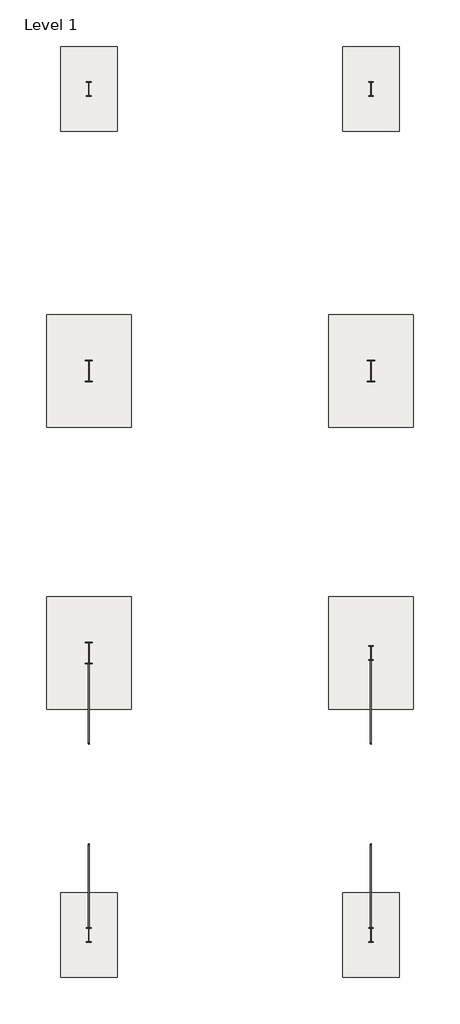
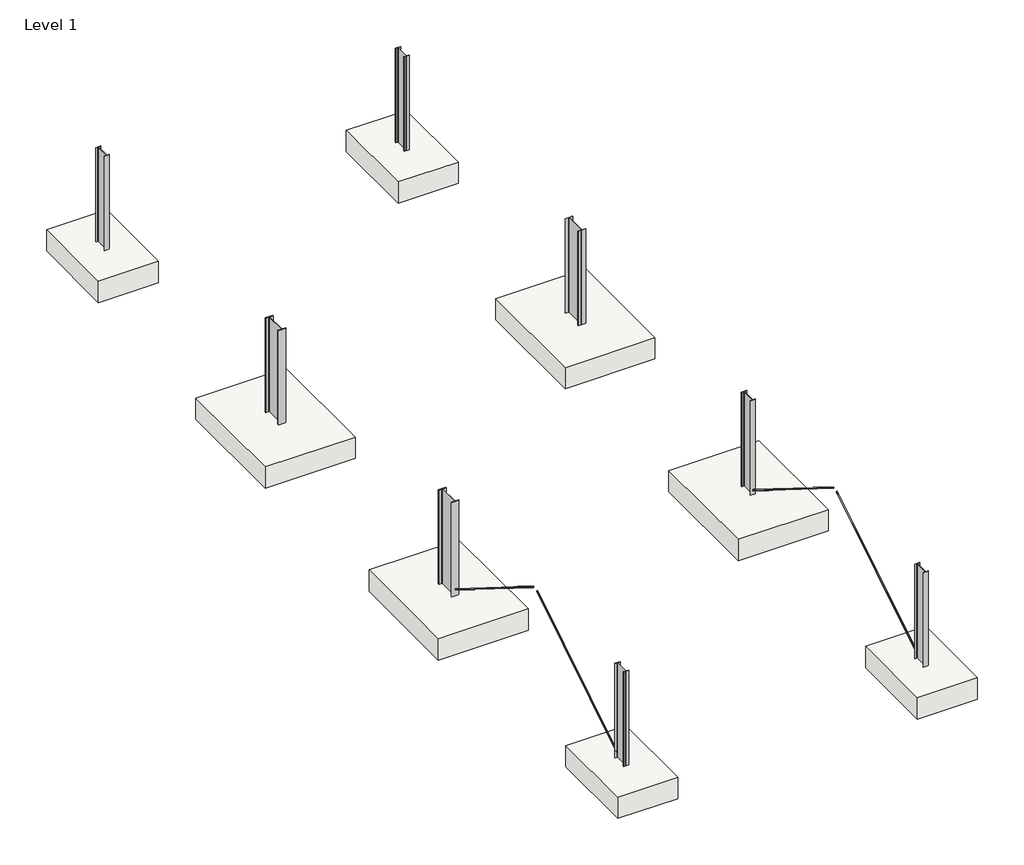
# One storey: 8 columns, 8 slabs, 4 members.
"""IFC4 building model written with IfcOpenShell, lengths in millimetres."""

import ifcopenshell
import ifcopenshell.guid

model = None  # the IFC model being written
_history = None  # IfcOwnerHistory: only IFC2X3 demands one
_inside = {}  # id of a spatial element -> (the spatial element, [elements in it])
_under = {}  # id of a project, library or spatial element -> (it, [spatial elements below it])
_declared = {}  # id of a project -> (the project, [libraries it declares])
_typed = {}  # id of a type object -> (the type object, [elements of that type])
_made_of = {}  # id of a material, layer set ... -> (it, [elements and type objects made of it])


def new_model(schema):
    """Start an empty IFC model of exactly this schema.

    Asked for "IFC4X3", IfcOpenShell would pick the latest addendum, in which some entities
    have other attributes; the version numbers below select the first issue.
    IFC2X3 requires an IfcOwnerHistory on every rooted entity: one is made here for all.
    """
    global model, _history
    if schema == "IFC4X3":
        model = ifcopenshell.file(schema_version=(4, 3, 0, 0))
    else:
        model = ifcopenshell.file(schema=schema)
    _inside.clear()
    _under.clear()
    _declared.clear()
    _typed.clear()
    _made_of.clear()
    _history = None
    if model.schema == "IFC2X3":
        org = make("IfcOrganization", Name="unknown")
        user = make(
            "IfcPersonAndOrganization",
            ThePerson=make("IfcPerson", FamilyName="unknown"),
            TheOrganization=org,
        )
        app = make(
            "IfcApplication",
            ApplicationDeveloper=org,
            Version="unknown",
            ApplicationFullName="unknown",
            ApplicationIdentifier="unknown",
        )
        _history = make(
            "IfcOwnerHistory",
            OwningUser=user,
            OwningApplication=app,
            ChangeAction="ADDED",
            CreationDate=0,
        )
    return model


def make(cls, **values):
    """One entity of the class cls with the attributes given. An attribute that is None is left unset."""
    return model.create_entity(
        cls, **{name: value for name, value in values.items() if value is not None}
    )


def rooted(cls, **values):
    """An entity with a GlobalId (a new one), such as an element, a storey or a relation."""
    return make(cls, GlobalId=ifcopenshell.guid.new(), OwnerHistory=_history, **values)


def si_unit(unit_type, name, prefix=None):
    """IfcSIUnit, for example si_unit("LENGTHUNIT", "METRE", prefix="MILLI")."""
    return make("IfcSIUnit", UnitType=unit_type, Prefix=prefix, Name=name)


def assignment(units):
    """IfcUnitAssignment: the units of a project."""
    return None if units is None else make("IfcUnitAssignment", Units=units)


def point(xyz):
    """IfcCartesianPoint."""
    return None if xyz is None else make("IfcCartesianPoint", Coordinates=xyz)


def direction(xyz):
    """IfcDirection."""
    return None if xyz is None else make("IfcDirection", DirectionRatios=xyz)


def frame(location, z_axis=None, x_axis=None):
    """IfcAxis2Placement3D, a coordinate frame: its origin and axes. An axis left out is left unset."""
    return make(
        "IfcAxis2Placement3D",
        Location=point(location),
        Axis=direction(z_axis),
        RefDirection=direction(x_axis),
    )


def frame_2d(location, x_axis=None):
    """IfcAxis2Placement2D, a coordinate frame in the plane: its origin and x axis."""
    return make(
        "IfcAxis2Placement2D", Location=point(location), RefDirection=direction(x_axis)
    )


def origin():
    """The frame at (0, 0, 0) with its axes left unset."""
    return frame((0.0, 0.0, 0.0))


def origin_with_axes():
    """The frame at (0, 0, 0) with the z axis (0, 0, 1) and the x axis (1, 0, 0) written out."""
    return frame((0.0, 0.0, 0.0), z_axis=(0.0, 0.0, 1.0), x_axis=(1.0, 0.0, 0.0))


def origin_2d():
    """The frame at (0, 0) in the plane with its x axis left unset."""
    return frame_2d((0.0, 0.0))


def place(relative_to, where):
    """IfcLocalPlacement: puts the frame where relative to a parent placement (None: the world)."""
    return make(
        "IfcLocalPlacement", PlacementRelTo=relative_to, RelativePlacement=where
    )


def context(
    kind, dimensions, precision=None, world=None, true_north=None, identifier=None
):
    """IfcGeometricRepresentationContext, for example the 3D "Model" context."""
    return make(
        "IfcGeometricRepresentationContext",
        ContextIdentifier=identifier,
        ContextType=kind,
        CoordinateSpaceDimension=dimensions,
        Precision=precision,
        WorldCoordinateSystem=world,
        TrueNorth=true_north,
    )


def project(units=None, contexts=None):
    """IfcProject with its units and contexts."""
    return rooted(
        "IfcProject",
        Name="project",
        RepresentationContexts=contexts,
        UnitsInContext=assignment(units),
    )


def spatial(cls, under=None, at=None, **own):
    """A site, building, storey or space (cls), placed at a placement, below another one or the project."""
    s = rooted(cls, ObjectPlacement=at, **own)
    if under is not None:
        _under.setdefault(under.id(), (under, []))[1].append(s)
    return s


def polyline(points):
    """IfcPolyline through the points."""
    return make("IfcPolyline", Points=[point(p) for p in points])


def circle_curve(where, radius):
    """IfcCircle in the frame where."""
    return make("IfcCircle", Position=where, Radius=radius)


def trimmed(basis, trim1, trim2, sense, master):
    """IfcTrimmedCurve: the piece of a basis curve between two trims."""
    return make(
        "IfcTrimmedCurve",
        BasisCurve=basis,
        Trim1=trim1,
        Trim2=trim2,
        SenseAgreement=sense,
        MasterRepresentation=master,
    )


def segment(curve, same_sense, transition):
    """IfcCompositeCurveSegment."""
    return make(
        "IfcCompositeCurveSegment",
        Transition=transition,
        SameSense=same_sense,
        ParentCurve=curve,
    )


def composite_curve(segments, self_intersect=None):
    """IfcCompositeCurve: segments joined end to end."""
    return make("IfcCompositeCurve", Segments=segments, SelfIntersect=self_intersect)


def outline(outer, holes=None, kind="AREA"):
    """IfcArbitraryClosedProfileDef: a profile drawn as a closed curve; with holes, ...WithVoids."""
    if holes is None:
        return make("IfcArbitraryClosedProfileDef", ProfileType=kind, OuterCurve=outer)
    return make(
        "IfcArbitraryProfileDefWithVoids",
        ProfileType=kind,
        OuterCurve=outer,
        InnerCurves=holes,
    )


def extrude(swept, where, along, depth):
    """IfcExtrudedAreaSolid: the profile swept, set in the frame where, extruded along a direction by depth."""
    return make(
        "IfcExtrudedAreaSolid",
        SweptArea=swept,
        Position=where,
        ExtrudedDirection=direction(along),
        Depth=depth,
    )


def shape(context_of_items, identifier, shape_type, items):
    """IfcShapeRepresentation: the items that make up one representation, for example the "Body"."""
    return make(
        "IfcShapeRepresentation",
        ContextOfItems=context_of_items,
        RepresentationIdentifier=identifier,
        RepresentationType=shape_type,
        Items=items,
    )


def source(mapping_origin, context_of_items, identifier, shape_type, items):
    """IfcRepresentationMap: a shape defined once, which mapped items show again and again."""
    return make(
        "IfcRepresentationMap",
        MappingOrigin=mapping_origin,
        MappedRepresentation=shape(context_of_items, identifier, shape_type, items),
    )


def transform(
    local_origin,
    x_axis=None,
    y_axis=None,
    z_axis=None,
    scale=None,
    scale2=None,
    scale3=None,
    uniform=True,
):
    """IfcCartesianTransformationOperator3D, or its non-uniform kind. x_axis, y_axis, z_axis: its Axis1, 2, 3."""
    if uniform:
        return make(
            "IfcCartesianTransformationOperator3D",
            Axis1=direction(x_axis),
            Axis2=direction(y_axis),
            LocalOrigin=point(local_origin),
            Scale=scale,
            Axis3=direction(z_axis),
        )
    return make(
        "IfcCartesianTransformationOperator3DnonUniform",
        Axis1=direction(x_axis),
        Axis2=direction(y_axis),
        LocalOrigin=point(local_origin),
        Scale=scale,
        Axis3=direction(z_axis),
        Scale2=scale2,
        Scale3=scale3,
    )


def mapped(mapping_source, mapping_target):
    """IfcMappedItem: shows the shape of a source again, moved by a transform."""
    return make(
        "IfcMappedItem", MappingSource=mapping_source, MappingTarget=mapping_target
    )


def made_of(thing, what):
    """Note that an element or type object is made of a material, layer set ...; save() writes the relation."""
    if what is not None:
        _made_of.setdefault(what.id(), (what, []))[1].append(thing)
    return thing


def element(
    cls,
    number,
    at=None,
    inside=None,
    cuts=None,
    type_object=None,
    material=None,
    context=None,
    identifier="Body",
    shape_type=None,
    held_by="IfcProductDefinitionShape",
    body=None,
    shapes=None,
    **own,
):
    """One element of the class cls, such as IfcWall. Its Tag is "e" and its number.

    at: its placement. inside: the storey or other place that contains it. cuts: it is an
    opening in that element (IfcRelVoidsElement). A single representation is given by context,
    identifier, shape_type and body (its items); several are given by shapes. held_by: the class
    of the entity that holds the representations. save() writes the other relations.
    """
    e = rooted(cls, Tag="e%d" % number, ObjectPlacement=at, **own)
    if body is not None:
        shapes = [shape(context, identifier, shape_type, body)]
    if shapes is not None:
        e.Representation = make(held_by, Representations=shapes)
    if inside is not None:
        _inside.setdefault(inside.id(), (inside, []))[1].append(e)
    if cuts is not None:
        rooted(
            "IfcRelVoidsElement", RelatingBuildingElement=cuts, RelatedOpeningElement=e
        )
    if type_object is not None:
        _typed.setdefault(type_object.id(), (type_object, []))[1].append(e)
    return made_of(e, material)


def aggregate(whole, parts):
    """IfcRelAggregates: a whole, such as a stair, and the parts it consists of."""
    return rooted("IfcRelAggregates", RelatingObject=whole, RelatedObjects=parts)


def save(model, path):
    """Write the relations noted so far, then the file.

    IfcRelAggregates (storeys below a building ...), IfcRelContainedInSpatialStructure (elements
    in a storey), IfcRelDefinesByType, IfcRelAssociatesMaterial and IfcRelDeclares: one each for
    every whole, place, type object, material and project.
    """
    for whole, parts in _under.values():
        aggregate(whole, parts)
    for where, things in _inside.values():
        rooted(
            "IfcRelContainedInSpatialStructure",
            RelatedElements=things,
            RelatingStructure=where,
        )
    for kind, things in _typed.values():
        rooted("IfcRelDefinesByType", RelatedObjects=things, RelatingType=kind)
    for what, things in _made_of.values():
        rooted("IfcRelAssociatesMaterial", RelatedObjects=things, RelatingMaterial=what)
    for by, libraries in _declared.values():
        rooted("IfcRelDeclares", RelatingContext=by, RelatedDefinitions=libraries)
    model.write(path)


def ub_universal_beams_column_ub305x102x25_fde077e1(model_context):
    return source(origin(), model_context, "Body", "SweptSolid", [
        extrude(outline(composite_curve([segment(polyline([(50.8, 152.55), (50.8, 145.55), (10.5, 145.55)]), True, "CONTINUOUS"), segment(trimmed(circle_curve(frame_2d((10.5, 137.95)), 7.6), [point((10.5, 145.55))], [point((2.9, 137.95))], True, "CARTESIAN"), True, "CONTINUOUS"), segment(polyline([(2.9, 137.95), (2.9, -137.95)]), True, "CONTINUOUS"), segment(trimmed(circle_curve(frame_2d((10.5, -137.95)), 7.6), [point((2.9, -137.95))], [point((10.5, -145.55))], True, "CARTESIAN"), True, "CONTINUOUS"), segment(polyline([(10.5, -145.55), (50.8, -145.55), (50.8, -152.55), (-50.8, -152.55), (-50.8, -145.55), (-10.5, -145.55)]), True, "CONTINUOUS"), segment(trimmed(circle_curve(frame_2d((-10.5, -137.95)), 7.6), [point((-10.5, -145.55))], [point((-2.9, -137.95))], True, "CARTESIAN"), True, "CONTINUOUS"), segment(polyline([(-2.9, -137.95), (-2.9, 137.95)]), True, "CONTINUOUS"), segment(trimmed(circle_curve(frame_2d((-10.5, 137.95)), 7.6), [point((-2.9, 137.95))], [point((-10.5, 145.55))], True, "CARTESIAN"), True, "CONTINUOUS"), segment(polyline([(-10.5, 145.55), (-50.8, 145.55), (-50.8, 152.55), (50.8, 152.55)]), True, "CONTINUOUS")], self_intersect=False)), origin_with_axes(), (0.0, 0.0, 1.0), 2000.0),
    ])


def ub_universal_beams_column_ub457x152x52_1aa4cf6f(model_context):
    return source(origin(), model_context, "Body", "SweptSolid", [
        extrude(outline(composite_curve([segment(polyline([(76.2, 224.9), (76.2, 214.0), (14.0, 214.0)]), True, "CONTINUOUS"), segment(trimmed(circle_curve(frame_2d((14.0, 203.8)), 10.2), [point((14.0, 214.0))], [point((3.8, 203.8))], True, "CARTESIAN"), True, "CONTINUOUS"), segment(polyline([(3.8, 203.8), (3.8, -203.8)]), True, "CONTINUOUS"), segment(trimmed(circle_curve(frame_2d((14.0, -203.8)), 10.2), [point((3.8, -203.8))], [point((14.0, -214.0))], True, "CARTESIAN"), True, "CONTINUOUS"), segment(polyline([(14.0, -214.0), (76.2, -214.0), (76.2, -224.9), (-76.2, -224.9), (-76.2, -214.0), (-14.0, -214.0)]), True, "CONTINUOUS"), segment(trimmed(circle_curve(frame_2d((-14.0, -203.8)), 10.2), [point((-14.0, -214.0))], [point((-3.8, -203.8))], True, "CARTESIAN"), True, "CONTINUOUS"), segment(polyline([(-3.8, -203.8), (-3.8, 203.8)]), True, "CONTINUOUS"), segment(trimmed(circle_curve(frame_2d((-14.0, 203.8)), 10.2), [point((-3.8, 203.8))], [point((-14.0, 214.0))], True, "CARTESIAN"), True, "CONTINUOUS"), segment(polyline([(-14.0, 214.0), (-76.2, 214.0), (-76.2, 224.9), (76.2, 224.9)]), True, "CONTINUOUS")], self_intersect=False)), origin_with_axes(), (0.0, 0.0, 1.0), 2000.0),
    ])


def circular_hollow_sections_chs21_3x3_2_132da75c(model_context):
    return source(origin(), model_context, "Body", "SweptSolid", [
        extrude(outline(composite_curve([segment(trimmed(circle_curve(origin_2d(), 10.65), [point((-10.65, 0.0))], [point((10.65, 0.0))], False, "CARTESIAN"), True, "CONTINUOUS"), segment(trimmed(circle_curve(origin_2d(), 10.65), [point((10.65, 0.0))], [point((-10.65, 0.0))], False, "CARTESIAN"), True, "CONTINUOUS")], self_intersect=False), holes=[composite_curve([segment(trimmed(circle_curve(origin_2d(), 7.45), [point((7.45, 0.0))], [point((-7.45, 0.0))], True, "CARTESIAN"), True, "CONTINUOUS"), segment(trimmed(circle_curve(origin_2d(), 7.45), [point((-7.45, 0.0))], [point((7.45, 0.0))], True, "CARTESIAN"), True, "CONTINUOUS")], self_intersect=False)]), frame((-1569.15, 0.0, 0.0), z_axis=(1.0, 0.0, 0.0), x_axis=(0.0, 1.0, 0.0)), (0.0, 0.0, 1.0), 3258.2),
    ])


def circular_hollow_sections_chs21_3x3_2_397a7a56(model_context):
    return source(origin(), model_context, "Body", "SweptSolid", [
        extrude(outline(composite_curve([segment(trimmed(circle_curve(origin_2d(), 10.65), [point((-10.65, 0.0))], [point((10.65, 0.0))], False, "CARTESIAN"), True, "CONTINUOUS"), segment(trimmed(circle_curve(origin_2d(), 10.65), [point((10.65, 0.0))], [point((-10.65, 0.0))], False, "CARTESIAN"), True, "CONTINUOUS")], self_intersect=False), holes=[composite_curve([segment(trimmed(circle_curve(origin_2d(), 7.45), [point((7.45, 0.0))], [point((-7.45, 0.0))], True, "CARTESIAN"), True, "CONTINUOUS"), segment(trimmed(circle_curve(origin_2d(), 7.45), [point((-7.45, 0.0))], [point((7.45, 0.0))], True, "CARTESIAN"), True, "CONTINUOUS")], self_intersect=False)]), frame((-1483.85, 0.0, 0.0), z_axis=(1.0, 0.0, 0.0), x_axis=(0.0, 1.0, 0.0)), (0.0, 0.0, 1.0), 3172.9),
    ])


def footing_rectangular_1800_x_1200_x_450mm_16ba7ea5(model_context):
    return source(origin(), model_context, "Body", "SweptSolid", [
        extrude(outline(polyline([(600.0, 900.0), (600.0, -900.0), (-600.0, -900.0), (-600.0, 900.0), (600.0, 900.0)])), frame((0.0, 0.0, -450.0), z_axis=(0.0, 0.0, 1.0), x_axis=(1.0, 0.0, 0.0)), (0.0, 0.0, 1.0), 450.0),
    ])


def footing_rectangular_2400_x_1800_x_450mm_039970dc(model_context):
    return source(origin(), model_context, "Body", "SweptSolid", [
        extrude(outline(polyline([(900.0, 1200.0), (900.0, -1200.0), (-900.0, -1200.0), (-900.0, 1200.0), (900.0, 1200.0)])), frame((0.0, 0.0, -450.0), z_axis=(0.0, 0.0, 1.0), x_axis=(1.0, 0.0, 0.0)), (0.0, 0.0, 1.0), 450.0),
    ])


model = new_model("IFC4")

# Units and contexts
model_context = context("Model", 3, world=origin())
ifc_project = project(units=[si_unit("LENGTHUNIT", "METRE", prefix="MILLI")], contexts=[model_context])

# Site, building, storey
site = spatial("IfcSite", under=ifc_project)
building = spatial("IfcBuilding", under=site)
storey = spatial("IfcBuildingStorey", under=building, Name="Level 1", Elevation=0.0)

# Columns
placement = place(None, origin())
ub_universal_beams_column_ub305x102x25_shape = ub_universal_beams_column_ub305x102x25_fde077e1(model_context)
element("IfcColumn", 1, ObjectType="UB-Universal Beams-Column : UB305x102x25", at=placement, inside=storey, context=model_context, shape_type="MappedRepresentation", body=[
    mapped(ub_universal_beams_column_ub305x102x25_shape, transform((-3383.1518909, 6686.3953161, 0.0), x_axis=(1.0, 0.0, 0.0), y_axis=(0.0, 1.0, 0.0), z_axis=(0.0, 0.0, 1.0))),
])
element("IfcColumn", 2, ObjectType="UB-Universal Beams-Column : UB305x102x25", at=placement, inside=storey, context=model_context, shape_type="MappedRepresentation", body=[
    mapped(ub_universal_beams_column_ub305x102x25_shape, transform((2616.8481091, 6686.3953161, 0.0), x_axis=(1.0, 0.0, 0.0), y_axis=(0.0, 1.0, 0.0), z_axis=(0.0, 0.0, 1.0))),
])
element("IfcColumn", 3, ObjectType="UB-Universal Beams-Column : UB305x102x25", at=placement, inside=storey, context=model_context, shape_type="MappedRepresentation", body=[
    mapped(ub_universal_beams_column_ub305x102x25_shape, transform((2616.8481091, -5313.6046839, 0.0), x_axis=(1.0, 0.0, 0.0), y_axis=(0.0, 1.0, 0.0), z_axis=(0.0, 0.0, 1.0))),
])
element("IfcColumn", 4, ObjectType="UB-Universal Beams-Column : UB305x102x25", at=placement, inside=storey, context=model_context, shape_type="MappedRepresentation", body=[
    mapped(ub_universal_beams_column_ub305x102x25_shape, transform((-3383.1518909, -11313.6046839, 0.0), x_axis=(1.0, 0.0, 0.0), y_axis=(0.0, 1.0, 0.0), z_axis=(0.0, 0.0, 1.0))),
])
element("IfcColumn", 5, ObjectType="UB-Universal Beams-Column : UB305x102x25", at=placement, inside=storey, context=model_context, shape_type="MappedRepresentation", body=[
    mapped(ub_universal_beams_column_ub305x102x25_shape, transform((2616.8481091, -11313.6046839, 0.0), x_axis=(1.0, 0.0, 0.0), y_axis=(0.0, 1.0, 0.0), z_axis=(0.0, 0.0, 1.0))),
])
ub_universal_beams_column_ub457x152x52_shape = ub_universal_beams_column_ub457x152x52_1aa4cf6f(model_context)
element("IfcColumn", 6, ObjectType="UB-Universal Beams-Column : UB457x152x52", at=placement, inside=storey, context=model_context, shape_type="MappedRepresentation", body=[
    mapped(ub_universal_beams_column_ub457x152x52_shape, transform((-3383.1518909, 686.3953161, 0.0), x_axis=(1.0, 0.0, 0.0), y_axis=(0.0, 1.0, 0.0), z_axis=(0.0, 0.0, 1.0))),
])
element("IfcColumn", 7, ObjectType="UB-Universal Beams-Column : UB457x152x52", at=placement, inside=storey, context=model_context, shape_type="MappedRepresentation", body=[
    mapped(ub_universal_beams_column_ub457x152x52_shape, transform((2616.8481091, 686.3953161, 0.0), x_axis=(1.0, 0.0, 0.0), y_axis=(0.0, 1.0, 0.0), z_axis=(0.0, 0.0, 1.0))),
])
element("IfcColumn", 8, ObjectType="UB-Universal Beams-Column : UB457x152x52", at=placement, inside=storey, context=model_context, shape_type="MappedRepresentation", body=[
    mapped(ub_universal_beams_column_ub457x152x52_shape, transform((-3383.1518909, -5313.6046839, 0.0), x_axis=(1.0, 0.0, 0.0), y_axis=(0.0, 1.0, 0.0), z_axis=(0.0, 0.0, 1.0))),
])

# Members
circular_hollow_sections_chs21_3x3_2_shape = circular_hollow_sections_chs21_3x3_2_132da75c(model_context)
element("IfcMember", 9, ObjectType="Circular Hollow Sections : CHS21.3x3.2", at=placement, inside=storey, context=model_context, shape_type="MappedRepresentation", body=[
    mapped(circular_hollow_sections_chs21_3x3_2_shape, transform((-3383.1518909, -9813.6046839, 936.5), x_axis=(0.0, 0.8482523645128853, 0.5295922262442104), y_axis=(-1.0, 0.0, 0.0), z_axis=(0.0, -0.5295922262442104, 0.8482523645128853))),
])
element("IfcMember", 10, ObjectType="Circular Hollow Sections : CHS21.3x3.2", at=placement, inside=storey, context=model_context, shape_type="MappedRepresentation", body=[
    mapped(circular_hollow_sections_chs21_3x3_2_shape, transform((2616.8481091, -9813.6046839, 936.5), x_axis=(0.0, 0.8482523645128854, 0.5295922262442104), y_axis=(-1.0, 0.0, 0.0), z_axis=(0.0, -0.5295922262442104, 0.8482523645128854))),
])
element("IfcMember", 11, ObjectType="Circular Hollow Sections : CHS21.3x3.2", at=placement, inside=storey, context=model_context, shape_type="MappedRepresentation", body=[
    mapped(circular_hollow_sections_chs21_3x3_2_shape, transform((2616.8481091, -6813.6046839, 936.5), x_axis=(0.0, -0.8482523645128853, 0.5295922262442104), y_axis=(1.0, 0.0, 0.0), z_axis=(0.0, 0.5295922262442104, 0.8482523645128853))),
])
circular_hollow_sections_chs21_3x3_2_2_shape = circular_hollow_sections_chs21_3x3_2_397a7a56(model_context)
element("IfcMember", 12, ObjectType="Circular Hollow Sections : CHS21.3x3.2", at=placement, inside=storey, context=model_context, shape_type="MappedRepresentation", body=[
    mapped(circular_hollow_sections_chs21_3x3_2_2_shape, transform((-3383.1518909, -6813.6046839, 936.5), x_axis=(0.0, -0.8482523645128853, 0.5295922262442104), y_axis=(1.0, 0.0, 0.0), z_axis=(0.0, 0.5295922262442104, 0.8482523645128853))),
])

# Slabs
footing_rectangular_1800_x_1200_x_450mm_shape = footing_rectangular_1800_x_1200_x_450mm_16ba7ea5(model_context)
element("IfcSlab", 13, ObjectType="Footing-Rectangular : 1800 x 1200 x 450mm", at=placement, inside=storey, context=model_context, shape_type="MappedRepresentation", body=[
    mapped(footing_rectangular_1800_x_1200_x_450mm_shape, transform((-3383.1518909, 6686.3953161, 0.0), x_axis=(1.0, 0.0, 0.0), y_axis=(0.0, 1.0, 0.0), z_axis=(0.0, 0.0, 1.0))),
])
element("IfcSlab", 14, ObjectType="Footing-Rectangular : 1800 x 1200 x 450mm", at=placement, inside=storey, context=model_context, shape_type="MappedRepresentation", body=[
    mapped(footing_rectangular_1800_x_1200_x_450mm_shape, transform((2616.8481091, 6686.3953161, 0.0), x_axis=(1.0, 0.0, 0.0), y_axis=(0.0, 1.0, 0.0), z_axis=(0.0, 0.0, 1.0))),
])
element("IfcSlab", 15, ObjectType="Footing-Rectangular : 1800 x 1200 x 450mm", at=placement, inside=storey, context=model_context, shape_type="MappedRepresentation", body=[
    mapped(footing_rectangular_1800_x_1200_x_450mm_shape, transform((-3383.1518909, -11313.6046839, 0.0), x_axis=(1.0, 0.0, 0.0), y_axis=(0.0, 1.0, 0.0), z_axis=(0.0, 0.0, 1.0))),
])
element("IfcSlab", 16, ObjectType="Footing-Rectangular : 1800 x 1200 x 450mm", at=placement, inside=storey, context=model_context, shape_type="MappedRepresentation", body=[
    mapped(footing_rectangular_1800_x_1200_x_450mm_shape, transform((2616.8481091, -11313.6046839, 0.0), x_axis=(1.0, 0.0, 0.0), y_axis=(0.0, 1.0, 0.0), z_axis=(0.0, 0.0, 1.0))),
])
footing_rectangular_2400_x_1800_x_450mm_shape = footing_rectangular_2400_x_1800_x_450mm_039970dc(model_context)
element("IfcSlab", 17, ObjectType="Footing-Rectangular : 2400 x 1800 x 450mm", at=placement, inside=storey, context=model_context, shape_type="MappedRepresentation", body=[
    mapped(footing_rectangular_2400_x_1800_x_450mm_shape, transform((-3383.1518909, 686.3953161, 0.0), x_axis=(1.0, 0.0, 0.0), y_axis=(0.0, 1.0, 0.0), z_axis=(0.0, 0.0, 1.0))),
])
element("IfcSlab", 18, ObjectType="Footing-Rectangular : 2400 x 1800 x 450mm", at=placement, inside=storey, context=model_context, shape_type="MappedRepresentation", body=[
    mapped(footing_rectangular_2400_x_1800_x_450mm_shape, transform((-3383.1518909, -5313.6046839, 0.0), x_axis=(1.0, 0.0, 0.0), y_axis=(0.0, 1.0, 0.0), z_axis=(0.0, 0.0, 1.0))),
])
element("IfcSlab", 19, ObjectType="Footing-Rectangular : 2400 x 1800 x 450mm", at=placement, inside=storey, context=model_context, shape_type="MappedRepresentation", body=[
    mapped(footing_rectangular_2400_x_1800_x_450mm_shape, transform((2616.8481091, 686.3953161, 0.0), x_axis=(1.0, 0.0, 0.0), y_axis=(0.0, 1.0, 0.0), z_axis=(0.0, 0.0, 1.0))),
])
element("IfcSlab", 20, ObjectType="Footing-Rectangular : 2400 x 1800 x 450mm", at=placement, inside=storey, context=model_context, shape_type="MappedRepresentation", body=[
    mapped(footing_rectangular_2400_x_1800_x_450mm_shape, transform((2616.8481091, -5313.6046839, 0.0), x_axis=(1.0, 0.0, 0.0), y_axis=(0.0, 1.0, 0.0), z_axis=(0.0, 0.0, 1.0))),
])

save(model, "model.ifc")

# Revit data of these elements
# Project information
#   Project Issue Date = "Issue Date"
#   Project Status = "Project Status"
#   Client Name = "Owner"
#   Project Address = "Enter address here"
#   Project Name = "Project Name"
#   Project Number = "Project Number"
# Grids (mm)
#   "1": line (-3383.152, -12746.234) -> (-3383.152, 14200.848)
#   "2": line (2616.848, -12746.234) -> (2616.848, 14200.848)
#   "A": line (4209.211, -11313.605) -> (-3537.295, -11313.605)
#   "E": line (4209.211, -5307.957) -> (-3383.152, -5307.957)
#   "F": line (4209.211, 686.395) -> (-3383.152, 686.395)
# Type "UB-Universal Beams-Column : UB305x102x25"
#   Section Name Key = "UB305X102X25"
#   Width = 10.16 cm
#   Web Thickness = 0.58 cm
#   Web Fillet = 0.76 cm
#   Warping Constant = 27300.0 cm⁶
#   Torsional Moment of Inertia = 4.77 cm⁴
#   Section Area = 31.6 cm²
#   Plastic Modulus weak axis = 39.0 cm³
#   Plastic Modulus strong axis = 342.0 cm³
#   Nominal Weight = 24.7999 kgf/m
#   Moment of Inertia weak axis = 123.00 cm⁴
#   Moment of Inertia strong axis = 4455.00 cm⁴
#   Height = 30.51 cm
#   Flange Thickness = 0.7 cm
#   Elastic Modulus weak axis = 24.2 cm³
#   Elastic Modulus strong axis = 292.0 cm³
#   Centroid Vertical = 15.255 cm
#   Centroid Horizontal = 5.08 cm
#   Bolt Spacing = 5.4 cm
#   Structural Material [instance default] = Metal - Steel 43-275
#   Type Comments = ""
#   Assembly Code = ""
# Type "UB-Universal Beams-Column : UB457x152x52"
#   Section Name Key = "UB457X152X52"
#   Width = 15.24 cm
#   Web Thickness = 0.76 cm
#   Web Fillet = 1.02 cm
#   Warping Constant = 311000.0 cm⁶
#   Torsional Moment of Inertia = 21.40 cm⁴
#   Section Area = 66.6 cm²
#   Plastic Modulus weak axis = 133.0 cm³
#   Plastic Modulus strong axis = 1096.0 cm³
#   Nominal Weight = 52.2998 kgf/m
#   Moment of Inertia weak axis = 645.00 cm⁴
#   Moment of Inertia strong axis = 21369.00 cm⁴
#   Height = 44.98 cm
#   Flange Thickness = 1.09 cm
#   Elastic Modulus weak axis = 85.0 cm³
#   Elastic Modulus strong axis = 950.0 cm³
#   Centroid Vertical = 22.49 cm
#   Centroid Horizontal = 7.62 cm
#   Bolt Spacing = 9.0 cm
#   Structural Material [instance default] = Metal - Steel 43-275
#   Type Comments = ""
#   Assembly Code = ""
# Type "Circular Hollow Sections : CHS21.3x3.2"
#   Section Name Key = "Ch21.3x3.2"
#   Wall Nominal Thickness = 0.32 cm
#   Wall Design Thickness = 0.32 cm
#   Torsional Moment of Inertia = 1.54 cm⁴
#   Torsional Modulus = 1.44 cm³
#   Section Area = 1.82 cm²
#   Plastic Modulus strong axis = 1.06 cm³
#   Perimeter = 0.067 m²/m
#   Nominal Weight = 1.42999 kgf/m
#   Moment of Inertia strong axis = 0.768 cm⁴
#   Length [instance default] = 1500 mm
#   Elastic Modulus strong axis = 0.722 cm³
#   Diameter = 2.13 cm
#   Centroid Vertical = 1.065 cm
#   Centroid Horizontal = 1.065 cm
#   Structural Material [instance default] = Metal - Steel 50-355
#   Type Comments = ""
#   Assembly Code = ""
# Type "Footing-Rectangular : 1800 x 1200 x 450mm"
#   Width = 1200 mm
#   Length = 1800 mm
#   Foundation Thickness = 450 mm
#   Structural Material [instance default] = Concrete - Cast-in-Place Concrete
#   Assembly Code = ""
# Type "Footing-Rectangular : 2400 x 1800 x 450mm"
#   Width = 1800 mm
#   Length = 2400 mm
#   Foundation Thickness = 450 mm
#   Structural Material [instance default] = Concrete - Cast-in-Place Concrete
#   Assembly Code = ""
# Elements 1, 2, 3, 4, 5 (IfcColumn, "UB-Universal Beams-Column : UB305x102x25")
#   Structural Material = Metal - Steel 43-275
#   Phase Created = New Construction
#   Materials on its faces: "Metal - Steel 43-275"
# Elements 6, 7, 8 (IfcColumn, "UB-Universal Beams-Column : UB457x152x52")
#   Structural Material = Metal - Steel 43-275
#   Phase Created = New Construction
#   Materials on its faces: "Metal - Steel 43-275"
# Elements 9, 10, 11, 12 (IfcMember, "Circular Hollow Sections : CHS21.3x3.2")
#   Structural Material = Metal - Steel 43-275
#   Phase Created = New Construction
#   Materials on its faces: "Metal - Steel 43-275"
# Elements 13, 14, 15, 16 (IfcSlab, "Footing-Rectangular : 1800 x 1200 x 450mm")
#   Structural Material = Concrete - Cast-in-Place Concrete
#   Phase Created = New Construction
#   Materials on its faces: "Concrete - Cast-in-Place Concrete"
# Elements 17, 18, 19, 20 (IfcSlab, "Footing-Rectangular : 2400 x 1800 x 450mm")
#   Structural Material = Concrete - Cast-in-Place Concrete
#   Phase Created = New Construction
#   Materials on its faces: "Concrete - Cast-in-Place Concrete"
# Materials
#   "Metal - Steel 43-275": class "Metal", colour RGB 247 247 247, transparency 0, Cost = 0
#   "Metal - Steel 50-355": class "Metal", colour RGB 247 247 247, transparency 0, Cost = 0
#   "Concrete - Cast-in-Place Concrete": class "Concrete", colour RGB 192 192 192, transparency 0, Cost = 0
